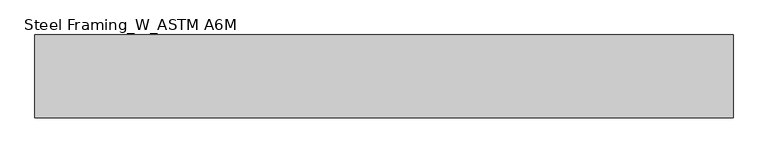
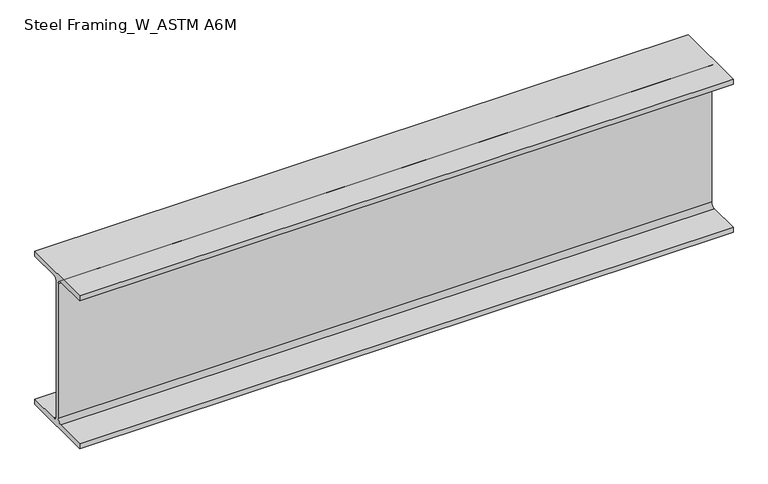
"""IFC4 building model written with IfcOpenShell, lengths in millimetres: beam geometry, Steel Framing_W_ASTM A6M : H_SB_AR_S02_W360x51_G3."""

from ifc_helpers import new_model, si_unit, point, frame, frame_2d, origin, place, context, project, spatial, polyline, circle_curve, trimmed, segment, composite_curve, outline, extrude, source, transform, mapped, element, save


def steel_framing_w_astm_a6m_0ec37d14(model_context):
    return source(origin(), model_context, "Body", "SweptSolid", [
        extrude(outline(composite_curve([segment(polyline([(85.5, -166.4), (85.5, -178.0), (-85.5, -178.0), (-85.5, -166.4), (-13.72, -166.4)]), True, "CONTINUOUS"), segment(trimmed(circle_curve(frame_2d((-13.72, -156.3)), 10.1), [point((-13.72, -166.4))], [point((-3.62, -156.3))], True, "CARTESIAN"), True, "CONTINUOUS"), segment(polyline([(-3.62, -156.3), (-3.62, 156.3)]), True, "CONTINUOUS"), segment(trimmed(circle_curve(frame_2d((-13.72, 156.3)), 10.1), [point((-3.62, 156.3))], [point((-13.72, 166.4))], True, "CARTESIAN"), True, "CONTINUOUS"), segment(polyline([(-13.72, 166.4), (-85.5, 166.4), (-85.5, 178.0), (85.5, 178.0), (85.5, 166.4), (13.72, 166.4)]), True, "CONTINUOUS"), segment(trimmed(circle_curve(frame_2d((13.72, 156.3)), 10.1), [point((13.72, 166.4))], [point((3.62, 156.3))], True, "CARTESIAN"), True, "CONTINUOUS"), segment(polyline([(3.62, 156.3), (3.62, -156.3)]), True, "CONTINUOUS"), segment(trimmed(circle_curve(frame_2d((13.72, -156.3)), 10.1), [point((3.62, -156.3))], [point((13.72, -166.4))], True, "CARTESIAN"), True, "CONTINUOUS"), segment(polyline([(13.72, -166.4), (85.5, -166.4)]), True, "CONTINUOUS")], self_intersect=False)), frame((-553.8, 0.0, 0.0), z_axis=(1.0, 0.0, 0.0), x_axis=(0.0, 1.0, 0.0)), (0.0, 0.0, 1.0), 1439.3),
    ])


if __name__ == "__main__":
    model = new_model("IFC4")
    model_context = context("Model", 3, world=origin())
    ifc_project = project(units=[si_unit("LENGTHUNIT", "METRE", prefix="MILLI")], contexts=[model_context])
    site = spatial("IfcSite", under=ifc_project)
    building = spatial("IfcBuilding", under=site)
    placement = place(None, origin())
    steel_framing_w_astm_a6m_shape = steel_framing_w_astm_a6m_0ec37d14(model_context)
    element("IfcBeam", 1, ObjectType="Steel Framing_W_ASTM A6M : H_SB_AR_S02_W360x51_G3", at=placement, inside=building, context=model_context, shape_type="MappedRepresentation", body=[
        mapped(steel_framing_w_astm_a6m_shape, transform((0.0, 0.0, 0.0), x_axis=(1.0, 0.0, 0.0), y_axis=(0.0, 1.0, 0.0), z_axis=(0.0, 0.0, 1.0))),
    ])
    save(model, "model.ifc")

# Revit data of these elements
# Type "Steel Framing_W_ASTM A6M : H_SB_AR_S02_W360x51_G3"
#   Type Mark = "G3"
#   Section Name Key = "W14x34"
#   Width = 17.1 cm
#   Web Thickness = 0.724 cm
#   Web Fillet = 1.01 cm
#   Warping Constant = 287000.0 cm⁶
#   Torsional Moment of Inertia = 23.70 cm⁴
#   Section Area = 64.5 cm²
#   Plastic Modulus weak axis = 174.0 cm³
#   Plastic Modulus strong axis = 895.0 cm³
#   Perimeter = 1.36 m²/m
#   Nominal Weight = 51.00 kgf/m
#   Moment of Inertia weak axis = 970.00 cm⁴
#   Moment of Inertia strong axis = 14200.00 cm⁴
#   Height = 35.6 cm
#   Flange Thickness = 1.16 cm
#   Elastic Modulus weak axis = 113.0 cm³
#   Elastic Modulus strong axis = 796.0 cm³
#   Centroid Vertical = 17.8 cm
#   Centroid Horizontal = 8.55 cm
#   Length [instance default] = 1500 mm
#   Structural Material [instance default] = Steel, 45-345
#   Bolt Spacing = 0
#   Assembly Code = ""
# Element 1 (IfcBeam, "Steel Framing_W_ASTM A6M : H_SB_AR_S02_W360x51_G3")
#   Materials on its faces: "Steel, 45-345"
# Materials
#   "Steel, 45-345": class "Metal", colour RGB 189 187 185, transparency 0, Description = "Steel 345 MPa", Cost = 0
